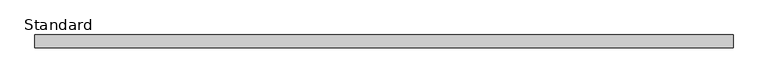
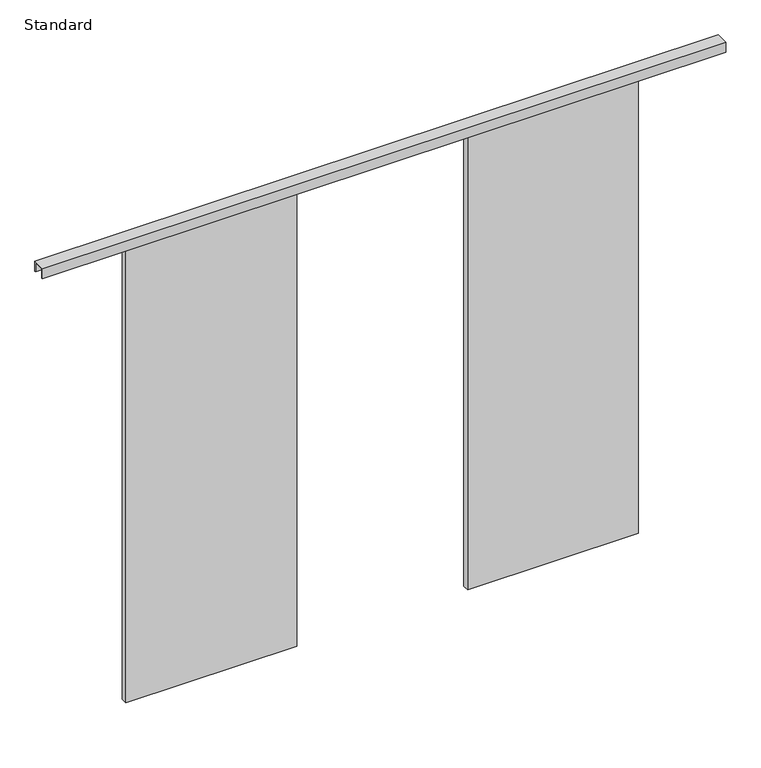
"""IFC4 building model written with IfcOpenShell, lengths in millimetres: plate geometry, Türelement 2-flg - Schiebeflügel : Standard."""

from ifc_helpers import new_model, si_unit, frame, origin, origin_with_axes, place, context, project, spatial, polyline, outline, extrude, source, transform, mapped, element, save


def standard_dba1ab43(model_context):
    return source(origin(), model_context, "Body", "SweptSolid", [
        extrude(outline(polyline([(1200.0, -100.0), (1200.0, -130.0), (400.0, -130.0), (400.0, -100.0), (1200.0, -100.0)])), origin_with_axes(), (0.0, 0.0, 1.0), 2250.0),
        extrude(outline(polyline([(-400.0, -100.0), (-400.0, -130.0), (-1200.0, -130.0), (-1200.0, -100.0), (-400.0, -100.0)])), origin_with_axes(), (0.0, 0.0, 1.0), 2250.0),
        extrude(outline(polyline([(-140.0, 2295.0), (-140.0, 2250.0), (-145.0, 2250.0), (-145.0, 2300.0), (-85.0, 2300.0), (-85.0, 2250.0), (-90.0, 2250.0), (-90.0, 2295.0), (-140.0, 2295.0)])), frame((-1600.0, 0.0, 0.0), z_axis=(1.0, 0.0, 0.0), x_axis=(0.0, 1.0, 0.0)), (0.0, 0.0, 1.0), 3200.0),
    ])


if __name__ == "__main__":
    model = new_model("IFC4")
    model_context = context("Model", 3, world=origin())
    ifc_project = project(units=[si_unit("LENGTHUNIT", "METRE", prefix="MILLI")], contexts=[model_context])
    site = spatial("IfcSite", under=ifc_project)
    building = spatial("IfcBuilding", under=site)
    placement = place(None, origin())
    standard_shape = standard_dba1ab43(model_context)
    element("IfcPlate", 1, ObjectType="Türelement 2-flg - Schiebeflügel : Standard", at=placement, inside=building, context=model_context, shape_type="MappedRepresentation", body=[
        mapped(standard_shape, transform((0.0, 0.0, 0.0), x_axis=(1.0, 0.0, 0.0), y_axis=(0.0, 1.0, 0.0), z_axis=(0.0, 0.0, 1.0))),
    ])
    save(model, "model.ifc")

# Revit data of these elements
# Type "Türelement 2-flg - Schiebeflügel : Standard"
#   Construction Type Id = "GSP4R"
#   Analytic Construction = "1/8 Zoll Pilkington-Verglasung einfach"
#   Visual Light Transmittance = 0.9
#   Thermal Resistance (R) = 0.270117 (m²·K)/W
#   Solar Heat Gain Coefficient = 0.86
#   Öffnungswert [instance default] = 0.400 m
#   Heat Transfer Coefficient (U) = 6.7069 W/(m²·K)
#   Länge Schiene [instance default] = 3.200 m
#   Halbe Breite [instance default] = 0.800 m
#   Versatz zur Achse [instance default] = 0.100 m
#   Gesamtbreite Tür [instance default] = 1.600 m
#   Schiene anzeigen [instance default] = yes
#   Prozent [instance default] = 50
#   Geöffnet in % [instance default] = 50
#   Schiene [instance default] = none
#   Tür [instance default] = none
# Element 1 (IfcPlate, "Türelement 2-flg - Schiebeflügel : Standard")
#   Materials on its faces: "Glas"
# Materials
#   "Glas": class "Glas", colour RGB 0 0 255, transparency 0.75, Comments = "Render-Darstellung nicht aktualisiert ", Cost = 0
